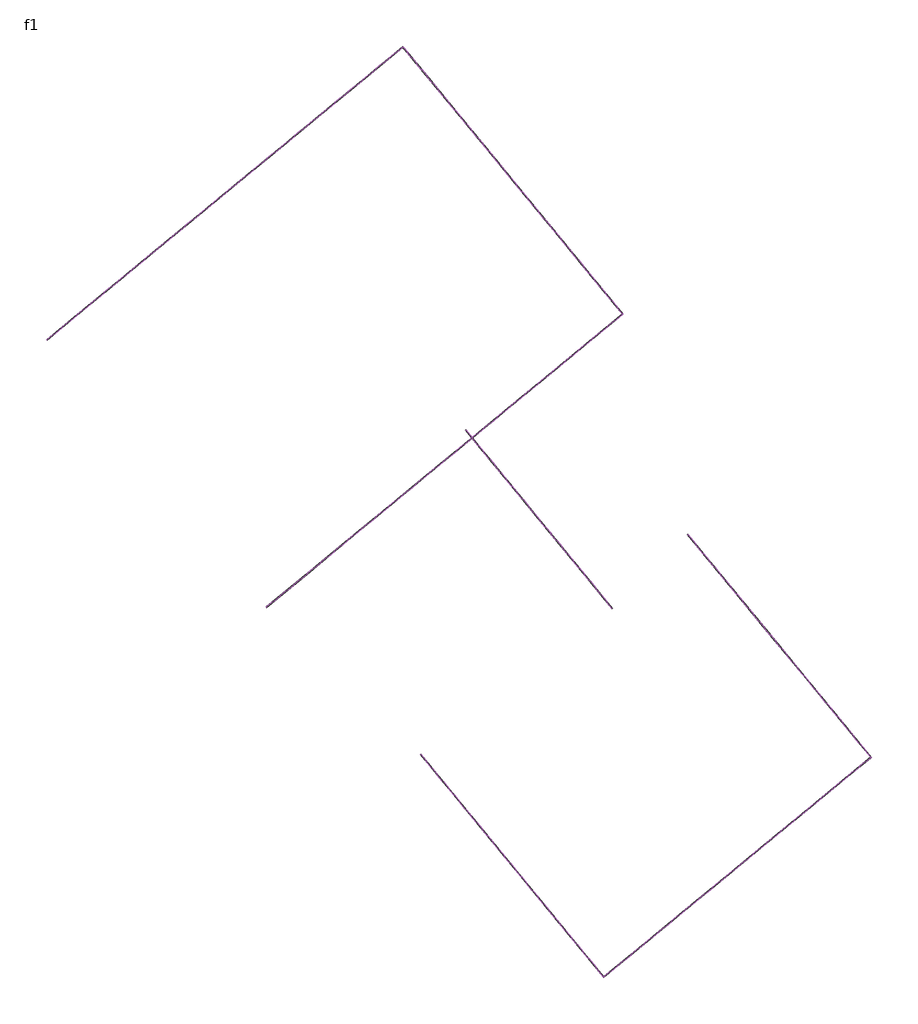
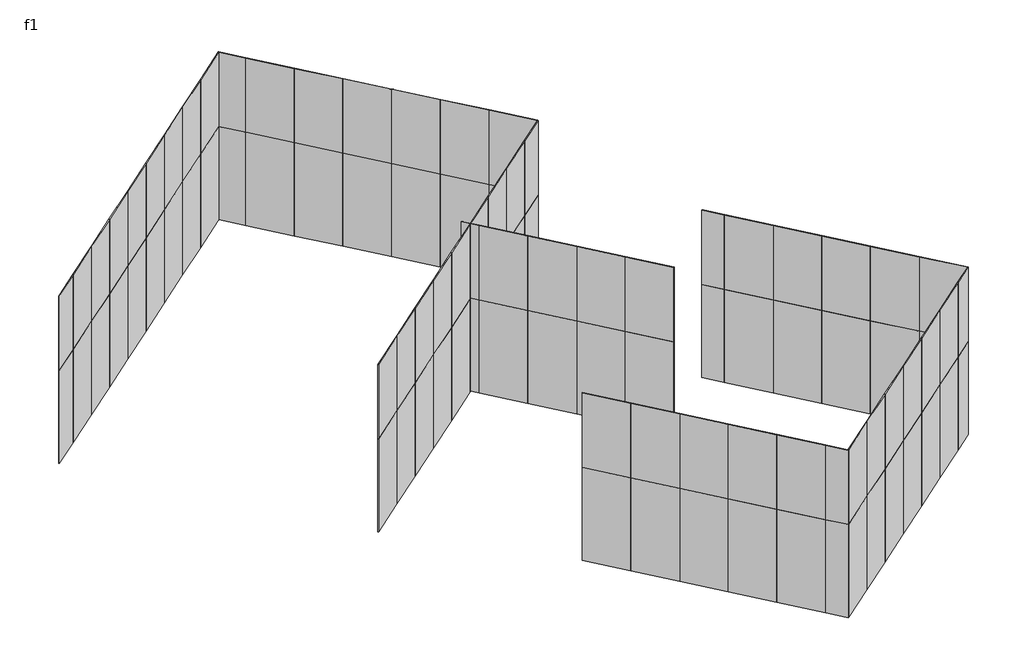
# One storey: 98 plates.
"""IFC4 building model written with IfcOpenShell, lengths in millimetres."""

import ifcopenshell
import ifcopenshell.guid

model = None  # the IFC model being written
_history = None  # IfcOwnerHistory: only IFC2X3 demands one
_inside = {}  # id of a spatial element -> (the spatial element, [elements in it])
_under = {}  # id of a project, library or spatial element -> (it, [spatial elements below it])
_declared = {}  # id of a project -> (the project, [libraries it declares])
_typed = {}  # id of a type object -> (the type object, [elements of that type])
_made_of = {}  # id of a material, layer set ... -> (it, [elements and type objects made of it])


def new_model(schema):
    """Start an empty IFC model of exactly this schema.

    Asked for "IFC4X3", IfcOpenShell would pick the latest addendum, in which some entities
    have other attributes; the version numbers below select the first issue.
    IFC2X3 requires an IfcOwnerHistory on every rooted entity: one is made here for all.
    """
    global model, _history
    if schema == "IFC4X3":
        model = ifcopenshell.file(schema_version=(4, 3, 0, 0))
    else:
        model = ifcopenshell.file(schema=schema)
    _inside.clear()
    _under.clear()
    _declared.clear()
    _typed.clear()
    _made_of.clear()
    _history = None
    if model.schema == "IFC2X3":
        org = make("IfcOrganization", Name="unknown")
        user = make(
            "IfcPersonAndOrganization",
            ThePerson=make("IfcPerson", FamilyName="unknown"),
            TheOrganization=org,
        )
        app = make(
            "IfcApplication",
            ApplicationDeveloper=org,
            Version="unknown",
            ApplicationFullName="unknown",
            ApplicationIdentifier="unknown",
        )
        _history = make(
            "IfcOwnerHistory",
            OwningUser=user,
            OwningApplication=app,
            ChangeAction="ADDED",
            CreationDate=0,
        )
    return model


def make(cls, **values):
    """One entity of the class cls with the attributes given. An attribute that is None is left unset."""
    return model.create_entity(
        cls, **{name: value for name, value in values.items() if value is not None}
    )


def rooted(cls, **values):
    """An entity with a GlobalId (a new one), such as an element, a storey or a relation."""
    return make(cls, GlobalId=ifcopenshell.guid.new(), OwnerHistory=_history, **values)


def si_unit(unit_type, name, prefix=None):
    """IfcSIUnit, for example si_unit("LENGTHUNIT", "METRE", prefix="MILLI")."""
    return make("IfcSIUnit", UnitType=unit_type, Prefix=prefix, Name=name)


def assignment(units):
    """IfcUnitAssignment: the units of a project."""
    return None if units is None else make("IfcUnitAssignment", Units=units)


def point(xyz):
    """IfcCartesianPoint."""
    return None if xyz is None else make("IfcCartesianPoint", Coordinates=xyz)


def direction(xyz):
    """IfcDirection."""
    return None if xyz is None else make("IfcDirection", DirectionRatios=xyz)


def frame(location, z_axis=None, x_axis=None):
    """IfcAxis2Placement3D, a coordinate frame: its origin and axes. An axis left out is left unset."""
    return make(
        "IfcAxis2Placement3D",
        Location=point(location),
        Axis=direction(z_axis),
        RefDirection=direction(x_axis),
    )


def origin():
    """The frame at (0, 0, 0) with its axes left unset."""
    return frame((0.0, 0.0, 0.0))


def origin_with_axes():
    """The frame at (0, 0, 0) with the z axis (0, 0, 1) and the x axis (1, 0, 0) written out."""
    return frame((0.0, 0.0, 0.0), z_axis=(0.0, 0.0, 1.0), x_axis=(1.0, 0.0, 0.0))


def place(relative_to, where):
    """IfcLocalPlacement: puts the frame where relative to a parent placement (None: the world)."""
    return make(
        "IfcLocalPlacement", PlacementRelTo=relative_to, RelativePlacement=where
    )


def context(
    kind, dimensions, precision=None, world=None, true_north=None, identifier=None
):
    """IfcGeometricRepresentationContext, for example the 3D "Model" context."""
    return make(
        "IfcGeometricRepresentationContext",
        ContextIdentifier=identifier,
        ContextType=kind,
        CoordinateSpaceDimension=dimensions,
        Precision=precision,
        WorldCoordinateSystem=world,
        TrueNorth=true_north,
    )


def project(units=None, contexts=None):
    """IfcProject with its units and contexts."""
    return rooted(
        "IfcProject",
        Name="project",
        RepresentationContexts=contexts,
        UnitsInContext=assignment(units),
    )


def spatial(cls, under=None, at=None, **own):
    """A site, building, storey or space (cls), placed at a placement, below another one or the project."""
    s = rooted(cls, ObjectPlacement=at, **own)
    if under is not None:
        _under.setdefault(under.id(), (under, []))[1].append(s)
    return s


def polyline(points):
    """IfcPolyline through the points."""
    return make("IfcPolyline", Points=[point(p) for p in points])


def outline(outer, holes=None, kind="AREA"):
    """IfcArbitraryClosedProfileDef: a profile drawn as a closed curve; with holes, ...WithVoids."""
    if holes is None:
        return make("IfcArbitraryClosedProfileDef", ProfileType=kind, OuterCurve=outer)
    return make(
        "IfcArbitraryProfileDefWithVoids",
        ProfileType=kind,
        OuterCurve=outer,
        InnerCurves=holes,
    )


def extrude(swept, where, along, depth):
    """IfcExtrudedAreaSolid: the profile swept, set in the frame where, extruded along a direction by depth."""
    return make(
        "IfcExtrudedAreaSolid",
        SweptArea=swept,
        Position=where,
        ExtrudedDirection=direction(along),
        Depth=depth,
    )


def shape(context_of_items, identifier, shape_type, items):
    """IfcShapeRepresentation: the items that make up one representation, for example the "Body"."""
    return make(
        "IfcShapeRepresentation",
        ContextOfItems=context_of_items,
        RepresentationIdentifier=identifier,
        RepresentationType=shape_type,
        Items=items,
    )


def source(mapping_origin, context_of_items, identifier, shape_type, items):
    """IfcRepresentationMap: a shape defined once, which mapped items show again and again."""
    return make(
        "IfcRepresentationMap",
        MappingOrigin=mapping_origin,
        MappedRepresentation=shape(context_of_items, identifier, shape_type, items),
    )


def transform(
    local_origin,
    x_axis=None,
    y_axis=None,
    z_axis=None,
    scale=None,
    scale2=None,
    scale3=None,
    uniform=True,
):
    """IfcCartesianTransformationOperator3D, or its non-uniform kind. x_axis, y_axis, z_axis: its Axis1, 2, 3."""
    if uniform:
        return make(
            "IfcCartesianTransformationOperator3D",
            Axis1=direction(x_axis),
            Axis2=direction(y_axis),
            LocalOrigin=point(local_origin),
            Scale=scale,
            Axis3=direction(z_axis),
        )
    return make(
        "IfcCartesianTransformationOperator3DnonUniform",
        Axis1=direction(x_axis),
        Axis2=direction(y_axis),
        LocalOrigin=point(local_origin),
        Scale=scale,
        Axis3=direction(z_axis),
        Scale2=scale2,
        Scale3=scale3,
    )


def mapped(mapping_source, mapping_target):
    """IfcMappedItem: shows the shape of a source again, moved by a transform."""
    return make(
        "IfcMappedItem", MappingSource=mapping_source, MappingTarget=mapping_target
    )


def made_of(thing, what):
    """Note that an element or type object is made of a material, layer set ...; save() writes the relation."""
    if what is not None:
        _made_of.setdefault(what.id(), (what, []))[1].append(thing)
    return thing


def element(
    cls,
    number,
    at=None,
    inside=None,
    cuts=None,
    type_object=None,
    material=None,
    context=None,
    identifier="Body",
    shape_type=None,
    held_by="IfcProductDefinitionShape",
    body=None,
    shapes=None,
    **own,
):
    """One element of the class cls, such as IfcWall. Its Tag is "e" and its number.

    at: its placement. inside: the storey or other place that contains it. cuts: it is an
    opening in that element (IfcRelVoidsElement). A single representation is given by context,
    identifier, shape_type and body (its items); several are given by shapes. held_by: the class
    of the entity that holds the representations. save() writes the other relations.
    """
    e = rooted(cls, Tag="e%d" % number, ObjectPlacement=at, **own)
    if body is not None:
        shapes = [shape(context, identifier, shape_type, body)]
    if shapes is not None:
        e.Representation = make(held_by, Representations=shapes)
    if inside is not None:
        _inside.setdefault(inside.id(), (inside, []))[1].append(e)
    if cuts is not None:
        rooted(
            "IfcRelVoidsElement", RelatingBuildingElement=cuts, RelatedOpeningElement=e
        )
    if type_object is not None:
        _typed.setdefault(type_object.id(), (type_object, []))[1].append(e)
    return made_of(e, material)


def aggregate(whole, parts):
    """IfcRelAggregates: a whole, such as a stair, and the parts it consists of."""
    return rooted("IfcRelAggregates", RelatingObject=whole, RelatedObjects=parts)


def save(model, path):
    """Write the relations noted so far, then the file.

    IfcRelAggregates (storeys below a building ...), IfcRelContainedInSpatialStructure (elements
    in a storey), IfcRelDefinesByType, IfcRelAssociatesMaterial and IfcRelDeclares: one each for
    every whole, place, type object, material and project.
    """
    for whole, parts in _under.values():
        aggregate(whole, parts)
    for where, things in _inside.values():
        rooted(
            "IfcRelContainedInSpatialStructure",
            RelatedElements=things,
            RelatingStructure=where,
        )
    for kind, things in _typed.values():
        rooted("IfcRelDefinesByType", RelatedObjects=things, RelatingType=kind)
    for what, things in _made_of.values():
        rooted("IfcRelAssociatesMaterial", RelatedObjects=things, RelatingMaterial=what)
    for by, libraries in _declared.values():
        rooted("IfcRelDeclares", RelatingContext=by, RelatedDefinitions=libraries)
    model.write(path)


def plate_0c29ff76(model_context):
    return source(origin(), model_context, "Body", "SweptSolid", [
        extrude(outline(polyline([(915.0, -12.5), (-915.0, -12.5), (-915.0, 12.5), (915.0, 12.5), (915.0, -12.5)])), origin_with_axes(), (0.0, 0.0, 1.0), 4000.0),
    ])


def plate_1e3715b7(model_context):
    return source(origin(), model_context, "Body", "SweptSolid", [
        extrude(outline(polyline([(510.0, -12.5), (-510.0, -12.5), (-510.0, 12.5), (510.0, 12.5), (510.0, -12.5)])), origin_with_axes(), (0.0, 0.0, 1.0), 4000.0),
    ])


def plate_751a20d5(model_context):
    return source(origin(), model_context, "Body", "SweptSolid", [
        extrude(outline(polyline([(915.0, -12.5), (-915.0, -12.5), (-915.0, 12.5), (915.0, 12.5), (915.0, -12.5)])), origin_with_axes(), (0.0, 0.0, 1.0), 3200.0),
    ])


def plate_eba9dd67(model_context):
    return source(origin(), model_context, "Body", "SweptSolid", [
        extrude(outline(polyline([(510.0, -12.5), (-510.0, -12.5), (-510.0, 12.5), (510.0, 12.5), (510.0, -12.5)])), origin_with_axes(), (0.0, 0.0, 1.0), 3200.0),
    ])


def plate_e4d7b700(model_context):
    return source(origin(), model_context, "Body", "SweptSolid", [
        extrude(outline(polyline([(680.0, -12.5), (-680.0, -12.5), (-680.0, 12.5), (680.0, 12.5), (680.0, -12.5)])), origin_with_axes(), (0.0, 0.0, 1.0), 4000.0),
    ])


def plate_81ff145c(model_context):
    return source(origin(), model_context, "Body", "SweptSolid", [
        extrude(outline(polyline([(680.0, -12.5), (-680.0, -12.5), (-680.0, 12.5), (680.0, 12.5), (680.0, -12.5)])), origin_with_axes(), (0.0, 0.0, 1.0), 3200.0),
    ])


def plate_147ead81(model_context):
    return source(origin(), model_context, "Body", "SweptSolid", [
        extrude(outline(polyline([(340.0, -12.5), (-340.0, -12.5), (-340.0, 12.5), (340.0, 12.5), (340.0, -12.5)])), origin_with_axes(), (0.0, 0.0, 1.0), 4000.0),
    ])


def plate_e10281fb(model_context):
    return source(origin(), model_context, "Body", "SweptSolid", [
        extrude(outline(polyline([(340.0, -12.5), (-340.0, -12.5), (-340.0, 12.5), (340.0, 12.5), (340.0, -12.5)])), origin_with_axes(), (0.0, 0.0, 1.0), 3200.0),
    ])


def plate_7a48b0fb(model_context):
    return source(origin(), model_context, "Body", "SweptSolid", [
        extrude(outline(polyline([(425.0, -12.5), (-425.0, -12.5), (-425.0, 12.5), (425.0, 12.5), (425.0, -12.5)])), origin_with_axes(), (0.0, 0.0, 1.0), 4000.0),
    ])


def plate_d5b4aa06(model_context):
    return source(origin(), model_context, "Body", "SweptSolid", [
        extrude(outline(polyline([(425.0, -12.5), (-425.0, -12.5), (-425.0, 12.5), (425.0, 12.5), (425.0, -12.5)])), origin_with_axes(), (0.0, 0.0, 1.0), 3200.0),
    ])


model = new_model("IFC4")

# Units and contexts
model_context = context("Model", 3, world=origin())
ifc_project = project(units=[si_unit("LENGTHUNIT", "METRE", prefix="MILLI")], contexts=[model_context])

# Site, building, storey
site = spatial("IfcSite", under=ifc_project)
building = spatial("IfcBuilding", under=site)
storey = spatial("IfcBuildingStorey", under=building, Name="f1", Elevation=3100.0)

# Plates
placement = place(None, origin())
plate_shape = plate_0c29ff76(model_context)
element("IfcPlate", 1, ObjectType="系统嵌板 : 玻璃", at=placement, inside=storey, context=model_context, shape_type="MappedRepresentation", body=[
    mapped(plate_shape, transform((-285.1263111, 24847.3639249, 3100.0), x_axis=(-0.6354332562848273, 0.7721557982734191, 0.0), y_axis=(-0.7721557982734191, -0.6354332562848273, 0.0), z_axis=(0.0, 0.0, 1.0))),
])
element("IfcPlate", 2, ObjectType="系统嵌板 : 玻璃", at=placement, inside=storey, context=model_context, shape_type="MappedRepresentation", body=[
    mapped(plate_shape, transform((-1447.9691701, 26260.4090358, 3100.0), x_axis=(-0.6354332562848273, 0.7721557982734191, 0.0), y_axis=(-0.7721557982734191, -0.6354332562848273, 0.0), z_axis=(0.0, 0.0, 1.0))),
])
element("IfcPlate", 3, ObjectType="系统嵌板 : 玻璃", at=placement, inside=storey, context=model_context, shape_type="MappedRepresentation", body=[
    mapped(plate_shape, transform((-2610.8120291, 27673.4541466, 3100.0), x_axis=(-0.6354332562848273, 0.7721557982734191, 0.0), y_axis=(-0.7721557982734191, -0.6354332562848273, 0.0), z_axis=(0.0, 0.0, 1.0))),
])
element("IfcPlate", 4, ObjectType="系统嵌板 : 玻璃", at=placement, inside=storey, context=model_context, shape_type="MappedRepresentation", body=[
    mapped(plate_shape, transform((-3773.6548881, 29086.4992575, 3100.0), x_axis=(-0.6354332562848273, 0.7721557982734191, 0.0), y_axis=(-0.7721557982734191, -0.6354332562848273, 0.0), z_axis=(0.0, 0.0, 1.0))),
])
element("IfcPlate", 5, ObjectType="系统嵌板 : 玻璃", at=placement, inside=storey, context=model_context, shape_type="MappedRepresentation", body=[
    mapped(plate_shape, transform((-4936.4977471, 30499.5443683, 3100.0), x_axis=(-0.6354332562848273, 0.7721557982734191, 0.0), y_axis=(-0.7721557982734191, -0.6354332562848273, 0.0), z_axis=(0.0, 0.0, 1.0))),
])
element("IfcPlate", 6, ObjectType="系统嵌板 : 玻璃", at=placement, inside=storey, context=model_context, shape_type="MappedRepresentation", body=[
    mapped(plate_shape, transform((-6099.3406061, 31912.5894791, 3100.0), x_axis=(-0.6354332562848273, 0.7721557982734191, 0.0), y_axis=(-0.7721557982734191, -0.6354332562848273, 0.0), z_axis=(0.0, 0.0, 1.0))),
])
element("IfcPlate", 7, ObjectType="系统嵌板 : 玻璃", at=placement, inside=storey, context=model_context, shape_type="MappedRepresentation", body=[
    mapped(plate_shape, transform((-8035.4265124, 32825.2895193, 3100.0), x_axis=(-0.7721557982734191, -0.6354332562848274, 0.0), y_axis=(0.6354332562848274, -0.7721557982734191, 0.0), z_axis=(0.0, 0.0, 1.0))),
])
element("IfcPlate", 8, ObjectType="系统嵌板 : 玻璃", at=placement, inside=storey, context=model_context, shape_type="MappedRepresentation", body=[
    mapped(plate_shape, transform((-9448.4716233, 31662.4466603, 3100.0), x_axis=(-0.7721557982734191, -0.6354332562848274, 0.0), y_axis=(0.6354332562848274, -0.7721557982734191, 0.0), z_axis=(0.0, 0.0, 1.0))),
])
element("IfcPlate", 9, ObjectType="系统嵌板 : 玻璃", at=placement, inside=storey, context=model_context, shape_type="MappedRepresentation", body=[
    mapped(plate_shape, transform((-10861.5167341, 30499.6038013, 3100.0), x_axis=(-0.7721557982734191, -0.6354332562848274, 0.0), y_axis=(0.6354332562848274, -0.7721557982734191, 0.0), z_axis=(0.0, 0.0, 1.0))),
])
element("IfcPlate", 10, ObjectType="系统嵌板 : 玻璃", at=placement, inside=storey, context=model_context, shape_type="MappedRepresentation", body=[
    mapped(plate_shape, transform((-12274.561845, 29336.7609423, 3100.0), x_axis=(-0.7721557982734191, -0.6354332562848274, 0.0), y_axis=(0.6354332562848274, -0.7721557982734191, 0.0), z_axis=(0.0, 0.0, 1.0))),
])
element("IfcPlate", 11, ObjectType="系统嵌板 : 玻璃", at=placement, inside=storey, context=model_context, shape_type="MappedRepresentation", body=[
    mapped(plate_shape, transform((-13687.6069558, 28173.9180833, 3100.0), x_axis=(-0.7721557982734191, -0.6354332562848274, 0.0), y_axis=(0.6354332562848274, -0.7721557982734191, 0.0), z_axis=(0.0, 0.0, 1.0))),
])
element("IfcPlate", 12, ObjectType="系统嵌板 : 玻璃", at=placement, inside=storey, context=model_context, shape_type="MappedRepresentation", body=[
    mapped(plate_shape, transform((-15100.6520666, 27011.0752243, 3100.0), x_axis=(-0.7721557982734191, -0.6354332562848274, 0.0), y_axis=(0.6354332562848274, -0.7721557982734191, 0.0), z_axis=(0.0, 0.0, 1.0))),
])
element("IfcPlate", 13, ObjectType="系统嵌板 : 玻璃", at=placement, inside=storey, context=model_context, shape_type="MappedRepresentation", body=[
    mapped(plate_shape, transform((-16513.6971775, 25848.2323653, 3100.0), x_axis=(-0.7721557982734191, -0.6354332562848274, 0.0), y_axis=(0.6354332562848274, -0.7721557982734191, 0.0), z_axis=(0.0, 0.0, 1.0))),
])
element("IfcPlate", 14, ObjectType="系统嵌板 : 玻璃", at=placement, inside=storey, context=model_context, shape_type="MappedRepresentation", body=[
    mapped(plate_shape, transform((-17926.7422883, 24685.3895063, 3100.0), x_axis=(-0.7721557982734191, -0.6354332562848274, 0.0), y_axis=(0.6354332562848274, -0.7721557982734191, 0.0), z_axis=(0.0, 0.0, 1.0))),
])
element("IfcPlate", 15, ObjectType="系统嵌板 : 玻璃", at=placement, inside=storey, context=model_context, shape_type="MappedRepresentation", body=[
    mapped(plate_shape, transform((-11351.6750986, 14555.3306985, 3100.0), x_axis=(0.772155798273419, 0.6354332562848274, 0.0), y_axis=(-0.6354332562848274, 0.772155798273419, 0.0), z_axis=(0.0, 0.0, 1.0))),
])
element("IfcPlate", 16, ObjectType="系统嵌板 : 玻璃", at=placement, inside=storey, context=model_context, shape_type="MappedRepresentation", body=[
    mapped(plate_shape, transform((-9938.6299877, 15718.1735575, 3100.0), x_axis=(0.772155798273419, 0.6354332562848274, 0.0), y_axis=(-0.6354332562848274, 0.772155798273419, 0.0), z_axis=(0.0, 0.0, 1.0))),
])
element("IfcPlate", 17, ObjectType="系统嵌板 : 玻璃", at=placement, inside=storey, context=model_context, shape_type="MappedRepresentation", body=[
    mapped(plate_shape, transform((-8525.5848769, 16881.0164165, 3100.0), x_axis=(0.772155798273419, 0.6354332562848274, 0.0), y_axis=(-0.6354332562848274, 0.772155798273419, 0.0), z_axis=(0.0, 0.0, 1.0))),
])
element("IfcPlate", 18, ObjectType="系统嵌板 : 玻璃", at=placement, inside=storey, context=model_context, shape_type="MappedRepresentation", body=[
    mapped(plate_shape, transform((-7112.539766, 18043.8592755, 3100.0), x_axis=(0.772155798273419, 0.6354332562848274, 0.0), y_axis=(-0.6354332562848274, 0.772155798273419, 0.0), z_axis=(0.0, 0.0, 1.0))),
])
element("IfcPlate", 19, ObjectType="系统嵌板 : 玻璃", at=placement, inside=storey, context=model_context, shape_type="MappedRepresentation", body=[
    mapped(plate_shape, transform((-5699.4946552, 19206.7021345, 3100.0), x_axis=(0.772155798273419, 0.6354332562848274, 0.0), y_axis=(-0.6354332562848274, 0.772155798273419, 0.0), z_axis=(0.0, 0.0, 1.0))),
])
element("IfcPlate", 20, ObjectType="系统嵌板 : 玻璃", at=placement, inside=storey, context=model_context, shape_type="MappedRepresentation", body=[
    mapped(plate_shape, transform((-4286.4495444, 20369.5449935, 3100.0), x_axis=(0.772155798273419, 0.6354332562848274, 0.0), y_axis=(-0.6354332562848274, 0.772155798273419, 0.0), z_axis=(0.0, 0.0, 1.0))),
])
element("IfcPlate", 21, ObjectType="系统嵌板 : 玻璃", at=placement, inside=storey, context=model_context, shape_type="MappedRepresentation", body=[
    mapped(plate_shape, transform((-2873.4044335, 21532.3878525, 3100.0), x_axis=(0.772155798273419, 0.6354332562848274, 0.0), y_axis=(-0.6354332562848274, 0.772155798273419, 0.0), z_axis=(0.0, 0.0, 1.0))),
])
element("IfcPlate", 22, ObjectType="系统嵌板 : 玻璃", at=placement, inside=storey, context=model_context, shape_type="MappedRepresentation", body=[
    mapped(plate_shape, transform((-1460.3593227, 22695.2307115, 3100.0), x_axis=(0.772155798273419, 0.6354332562848274, 0.0), y_axis=(-0.6354332562848274, 0.772155798273419, 0.0), z_axis=(0.0, 0.0, 1.0))),
])
element("IfcPlate", 23, ObjectType="系统嵌板 : 玻璃", at=placement, inside=storey, context=model_context, shape_type="MappedRepresentation", body=[
    mapped(plate_shape, transform((-640.1697835, 14643.621577, 3100.0), x_axis=(-0.6354332562848286, 0.7721557982734181, 0.0), y_axis=(-0.7721557982734181, -0.6354332562848286, 0.0), z_axis=(0.0, 0.0, 1.0))),
])
element("IfcPlate", 24, ObjectType="系统嵌板 : 玻璃", at=placement, inside=storey, context=model_context, shape_type="MappedRepresentation", body=[
    mapped(plate_shape, transform((-1803.0126425, 16056.6666878, 3100.0), x_axis=(-0.6354332562848286, 0.7721557982734181, 0.0), y_axis=(-0.7721557982734181, -0.6354332562848286, 0.0), z_axis=(0.0, 0.0, 1.0))),
])
element("IfcPlate", 25, ObjectType="系统嵌板 : 玻璃", at=placement, inside=storey, context=model_context, shape_type="MappedRepresentation", body=[
    mapped(plate_shape, transform((-2965.8555015, 17469.7117987, 3100.0), x_axis=(-0.6354332562848286, 0.7721557982734181, 0.0), y_axis=(-0.7721557982734181, -0.6354332562848286, 0.0), z_axis=(0.0, 0.0, 1.0))),
])
element("IfcPlate", 26, ObjectType="系统嵌板 : 玻璃", at=placement, inside=storey, context=model_context, shape_type="MappedRepresentation", body=[
    mapped(plate_shape, transform((-4128.6983605, 18882.7569095, 3100.0), x_axis=(-0.6354332562848286, 0.7721557982734181, 0.0), y_axis=(-0.7721557982734181, -0.6354332562848286, 0.0), z_axis=(0.0, 0.0, 1.0))),
])
element("IfcPlate", 27, ObjectType="系统嵌板 : 玻璃", at=placement, inside=storey, context=model_context, shape_type="MappedRepresentation", body=[
    mapped(plate_shape, transform((8328.6158526, 9478.9823292, 3100.0), x_axis=(-0.6354332562848274, 0.772155798273419, 0.0), y_axis=(-0.772155798273419, -0.6354332562848274, 0.0), z_axis=(0.0, 0.0, 1.0))),
])
element("IfcPlate", 28, ObjectType="系统嵌板 : 玻璃", at=placement, inside=storey, context=model_context, shape_type="MappedRepresentation", body=[
    mapped(plate_shape, transform((7165.7729936, 10892.02744, 3100.0), x_axis=(-0.6354332562848274, 0.772155798273419, 0.0), y_axis=(-0.772155798273419, -0.6354332562848274, 0.0), z_axis=(0.0, 0.0, 1.0))),
])
element("IfcPlate", 29, ObjectType="系统嵌板 : 玻璃", at=placement, inside=storey, context=model_context, shape_type="MappedRepresentation", body=[
    mapped(plate_shape, transform((6002.9301346, 12305.0725508, 3100.0), x_axis=(-0.6354332562848274, 0.772155798273419, 0.0), y_axis=(-0.772155798273419, -0.6354332562848274, 0.0), z_axis=(0.0, 0.0, 1.0))),
])
element("IfcPlate", 30, ObjectType="系统嵌板 : 玻璃", at=placement, inside=storey, context=model_context, shape_type="MappedRepresentation", body=[
    mapped(plate_shape, transform((4840.0872756, 13718.1176617, 3100.0), x_axis=(-0.6354332562848274, 0.772155798273419, 0.0), y_axis=(-0.772155798273419, -0.6354332562848274, 0.0), z_axis=(0.0, 0.0, 1.0))),
])
element("IfcPlate", 31, ObjectType="系统嵌板 : 玻璃", at=placement, inside=storey, context=model_context, shape_type="MappedRepresentation", body=[
    mapped(plate_shape, transform((3677.2444166, 15131.1627725, 3100.0), x_axis=(-0.6354332562848274, 0.772155798273419, 0.0), y_axis=(-0.772155798273419, -0.6354332562848274, 0.0), z_axis=(0.0, 0.0, 1.0))),
])
element("IfcPlate", 32, ObjectType="系统嵌板 : 玻璃", at=placement, inside=storey, context=model_context, shape_type="MappedRepresentation", body=[
    mapped(plate_shape, transform((350.6902583, 1728.6821278, 3100.0), x_axis=(0.7721557982734191, 0.6354332562848273, 0.0), y_axis=(-0.6354332562848273, 0.7721557982734191, 0.0), z_axis=(0.0, 0.0, 1.0))),
])
element("IfcPlate", 33, ObjectType="系统嵌板 : 玻璃", at=placement, inside=storey, context=model_context, shape_type="MappedRepresentation", body=[
    mapped(plate_shape, transform((1763.7353691, 2891.5249868, 3100.0), x_axis=(0.7721557982734191, 0.6354332562848273, 0.0), y_axis=(-0.6354332562848273, 0.7721557982734191, 0.0), z_axis=(0.0, 0.0, 1.0))),
])
element("IfcPlate", 34, ObjectType="系统嵌板 : 玻璃", at=placement, inside=storey, context=model_context, shape_type="MappedRepresentation", body=[
    mapped(plate_shape, transform((3176.78048, 4054.3678458, 3100.0), x_axis=(0.7721557982734191, 0.6354332562848273, 0.0), y_axis=(-0.6354332562848273, 0.7721557982734191, 0.0), z_axis=(0.0, 0.0, 1.0))),
])
element("IfcPlate", 35, ObjectType="系统嵌板 : 玻璃", at=placement, inside=storey, context=model_context, shape_type="MappedRepresentation", body=[
    mapped(plate_shape, transform((4589.8255908, 5217.2107048, 3100.0), x_axis=(0.7721557982734191, 0.6354332562848273, 0.0), y_axis=(-0.6354332562848273, 0.7721557982734191, 0.0), z_axis=(0.0, 0.0, 1.0))),
])
element("IfcPlate", 36, ObjectType="系统嵌板 : 玻璃", at=placement, inside=storey, context=model_context, shape_type="MappedRepresentation", body=[
    mapped(plate_shape, transform((6002.8707016, 6380.0535638, 3100.0), x_axis=(0.7721557982734191, 0.6354332562848273, 0.0), y_axis=(-0.6354332562848273, 0.7721557982734191, 0.0), z_axis=(0.0, 0.0, 1.0))),
])
element("IfcPlate", 37, ObjectType="系统嵌板 : 玻璃", at=placement, inside=storey, context=model_context, shape_type="MappedRepresentation", body=[
    mapped(plate_shape, transform((7415.9158125, 7542.8964228, 3100.0), x_axis=(0.7721557982734191, 0.6354332562848273, 0.0), y_axis=(-0.6354332562848273, 0.7721557982734191, 0.0), z_axis=(0.0, 0.0, 1.0))),
])
element("IfcPlate", 38, ObjectType="系统嵌板 : 玻璃", at=placement, inside=storey, context=model_context, shape_type="MappedRepresentation", body=[
    mapped(plate_shape, transform((-6128.7434305, 8162.2961256, 3100.0), x_axis=(0.6354332562848274, -0.7721557982734191, 0.0), y_axis=(0.7721557982734191, 0.6354332562848274, 0.0), z_axis=(0.0, 0.0, 1.0))),
])
element("IfcPlate", 39, ObjectType="系统嵌板 : 玻璃", at=placement, inside=storey, context=model_context, shape_type="MappedRepresentation", body=[
    mapped(plate_shape, transform((-4965.9005715, 6749.2510148, 3100.0), x_axis=(0.6354332562848274, -0.7721557982734191, 0.0), y_axis=(0.7721557982734191, 0.6354332562848274, 0.0), z_axis=(0.0, 0.0, 1.0))),
])
element("IfcPlate", 40, ObjectType="系统嵌板 : 玻璃", at=placement, inside=storey, context=model_context, shape_type="MappedRepresentation", body=[
    mapped(plate_shape, transform((-3803.0577125, 5336.2059039, 3100.0), x_axis=(0.6354332562848274, -0.7721557982734191, 0.0), y_axis=(0.7721557982734191, 0.6354332562848274, 0.0), z_axis=(0.0, 0.0, 1.0))),
])
element("IfcPlate", 41, ObjectType="系统嵌板 : 玻璃", at=placement, inside=storey, context=model_context, shape_type="MappedRepresentation", body=[
    mapped(plate_shape, transform((-2640.2148535, 3923.1607931, 3100.0), x_axis=(0.6354332562848274, -0.7721557982734191, 0.0), y_axis=(0.7721557982734191, 0.6354332562848274, 0.0), z_axis=(0.0, 0.0, 1.0))),
])
element("IfcPlate", 42, ObjectType="系统嵌板 : 玻璃", at=placement, inside=storey, context=model_context, shape_type="MappedRepresentation", body=[
    mapped(plate_shape, transform((-1477.3719945, 2510.1156823, 3100.0), x_axis=(0.6354332562848274, -0.7721557982734191, 0.0), y_axis=(0.7721557982734191, 0.6354332562848274, 0.0), z_axis=(0.0, 0.0, 1.0))),
])
plate_2_shape = plate_1e3715b7(model_context)
element("IfcPlate", 43, ObjectType="系统嵌板 : 玻璃", at=placement, inside=storey, context=model_context, shape_type="MappedRepresentation", body=[
    mapped(plate_2_shape, transform((-7004.8329963, 33012.9114917, 3100.0), x_axis=(-0.6354332562848273, 0.7721557982734191, 0.0), y_axis=(-0.7721557982734191, -0.6354332562848273, 0.0), z_axis=(0.0, 0.0, 1.0))),
])
element("IfcPlate", 44, ObjectType="系统嵌板 : 玻璃", at=placement, inside=storey, context=model_context, shape_type="MappedRepresentation", body=[
    mapped(plate_2_shape, transform((8516.237825, 8448.388813, 3100.0), x_axis=(0.7721557982734191, 0.6354332562848273, 0.0), y_axis=(-0.6354332562848273, 0.7721557982734191, 0.0), z_axis=(0.0, 0.0, 1.0))),
])
plate_3_shape = plate_751a20d5(model_context)
element("IfcPlate", 45, ObjectType="系统嵌板 : 玻璃", at=placement, inside=storey, context=model_context, shape_type="MappedRepresentation", body=[
    mapped(plate_3_shape, transform((-285.1263111, 24847.3639249, 7100.0), x_axis=(-0.6354332562848273, 0.7721557982734191, 0.0), y_axis=(-0.7721557982734191, -0.6354332562848273, 0.0), z_axis=(0.0, 0.0, 1.0))),
])
element("IfcPlate", 46, ObjectType="系统嵌板 : 玻璃", at=placement, inside=storey, context=model_context, shape_type="MappedRepresentation", body=[
    mapped(plate_3_shape, transform((-1447.9691701, 26260.4090358, 7100.0), x_axis=(-0.6354332562848273, 0.7721557982734191, 0.0), y_axis=(-0.7721557982734191, -0.6354332562848273, 0.0), z_axis=(0.0, 0.0, 1.0))),
])
element("IfcPlate", 47, ObjectType="系统嵌板 : 玻璃", at=placement, inside=storey, context=model_context, shape_type="MappedRepresentation", body=[
    mapped(plate_3_shape, transform((-2610.8120291, 27673.4541466, 7100.0), x_axis=(-0.6354332562848273, 0.7721557982734191, 0.0), y_axis=(-0.7721557982734191, -0.6354332562848273, 0.0), z_axis=(0.0, 0.0, 1.0))),
])
element("IfcPlate", 48, ObjectType="系统嵌板 : 玻璃", at=placement, inside=storey, context=model_context, shape_type="MappedRepresentation", body=[
    mapped(plate_3_shape, transform((-3773.6548881, 29086.4992575, 7100.0), x_axis=(-0.6354332562848273, 0.7721557982734191, 0.0), y_axis=(-0.7721557982734191, -0.6354332562848273, 0.0), z_axis=(0.0, 0.0, 1.0))),
])
element("IfcPlate", 49, ObjectType="系统嵌板 : 玻璃", at=placement, inside=storey, context=model_context, shape_type="MappedRepresentation", body=[
    mapped(plate_3_shape, transform((-4936.4977471, 30499.5443683, 7100.0), x_axis=(-0.6354332562848273, 0.7721557982734191, 0.0), y_axis=(-0.7721557982734191, -0.6354332562848273, 0.0), z_axis=(0.0, 0.0, 1.0))),
])
element("IfcPlate", 50, ObjectType="系统嵌板 : 玻璃", at=placement, inside=storey, context=model_context, shape_type="MappedRepresentation", body=[
    mapped(plate_3_shape, transform((-6099.3406061, 31912.5894791, 7100.0), x_axis=(-0.6354332562848273, 0.7721557982734191, 0.0), y_axis=(-0.7721557982734191, -0.6354332562848273, 0.0), z_axis=(0.0, 0.0, 1.0))),
])
element("IfcPlate", 51, ObjectType="系统嵌板 : 玻璃", at=placement, inside=storey, context=model_context, shape_type="MappedRepresentation", body=[
    mapped(plate_3_shape, transform((-8035.4265124, 32825.2895193, 7100.0), x_axis=(-0.7721557982734191, -0.6354332562848274, 0.0), y_axis=(0.6354332562848274, -0.7721557982734191, 0.0), z_axis=(0.0, 0.0, 1.0))),
])
element("IfcPlate", 52, ObjectType="系统嵌板 : 玻璃", at=placement, inside=storey, context=model_context, shape_type="MappedRepresentation", body=[
    mapped(plate_3_shape, transform((-9448.4716233, 31662.4466603, 7100.0), x_axis=(-0.7721557982734191, -0.6354332562848274, 0.0), y_axis=(0.6354332562848274, -0.7721557982734191, 0.0), z_axis=(0.0, 0.0, 1.0))),
])
element("IfcPlate", 53, ObjectType="系统嵌板 : 玻璃", at=placement, inside=storey, context=model_context, shape_type="MappedRepresentation", body=[
    mapped(plate_3_shape, transform((-10861.5167341, 30499.6038013, 7100.0), x_axis=(-0.7721557982734191, -0.6354332562848274, 0.0), y_axis=(0.6354332562848274, -0.7721557982734191, 0.0), z_axis=(0.0, 0.0, 1.0))),
])
element("IfcPlate", 54, ObjectType="系统嵌板 : 玻璃", at=placement, inside=storey, context=model_context, shape_type="MappedRepresentation", body=[
    mapped(plate_3_shape, transform((-12274.561845, 29336.7609423, 7100.0), x_axis=(-0.7721557982734191, -0.6354332562848274, 0.0), y_axis=(0.6354332562848274, -0.7721557982734191, 0.0), z_axis=(0.0, 0.0, 1.0))),
])
element("IfcPlate", 55, ObjectType="系统嵌板 : 玻璃", at=placement, inside=storey, context=model_context, shape_type="MappedRepresentation", body=[
    mapped(plate_3_shape, transform((-13687.6069558, 28173.9180833, 7100.0), x_axis=(-0.7721557982734191, -0.6354332562848274, 0.0), y_axis=(0.6354332562848274, -0.7721557982734191, 0.0), z_axis=(0.0, 0.0, 1.0))),
])
element("IfcPlate", 56, ObjectType="系统嵌板 : 玻璃", at=placement, inside=storey, context=model_context, shape_type="MappedRepresentation", body=[
    mapped(plate_3_shape, transform((-15100.6520666, 27011.0752243, 7100.0), x_axis=(-0.7721557982734191, -0.6354332562848274, 0.0), y_axis=(0.6354332562848274, -0.7721557982734191, 0.0), z_axis=(0.0, 0.0, 1.0))),
])
element("IfcPlate", 57, ObjectType="系统嵌板 : 玻璃", at=placement, inside=storey, context=model_context, shape_type="MappedRepresentation", body=[
    mapped(plate_3_shape, transform((-16513.6971775, 25848.2323653, 7100.0), x_axis=(-0.7721557982734191, -0.6354332562848274, 0.0), y_axis=(0.6354332562848274, -0.7721557982734191, 0.0), z_axis=(0.0, 0.0, 1.0))),
])
element("IfcPlate", 58, ObjectType="系统嵌板 : 玻璃", at=placement, inside=storey, context=model_context, shape_type="MappedRepresentation", body=[
    mapped(plate_3_shape, transform((-17926.7422883, 24685.3895063, 7100.0), x_axis=(-0.7721557982734191, -0.6354332562848274, 0.0), y_axis=(0.6354332562848274, -0.7721557982734191, 0.0), z_axis=(0.0, 0.0, 1.0))),
])
element("IfcPlate", 59, ObjectType="系统嵌板 : 玻璃", at=placement, inside=storey, context=model_context, shape_type="MappedRepresentation", body=[
    mapped(plate_3_shape, transform((-11351.6750986, 14555.3306985, 7100.0), x_axis=(0.772155798273419, 0.6354332562848274, 0.0), y_axis=(-0.6354332562848274, 0.772155798273419, 0.0), z_axis=(0.0, 0.0, 1.0))),
])
element("IfcPlate", 60, ObjectType="系统嵌板 : 玻璃", at=placement, inside=storey, context=model_context, shape_type="MappedRepresentation", body=[
    mapped(plate_3_shape, transform((-9938.6299877, 15718.1735575, 7100.0), x_axis=(0.772155798273419, 0.6354332562848274, 0.0), y_axis=(-0.6354332562848274, 0.772155798273419, 0.0), z_axis=(0.0, 0.0, 1.0))),
])
element("IfcPlate", 61, ObjectType="系统嵌板 : 玻璃", at=placement, inside=storey, context=model_context, shape_type="MappedRepresentation", body=[
    mapped(plate_3_shape, transform((-8525.5848769, 16881.0164165, 7100.0), x_axis=(0.772155798273419, 0.6354332562848274, 0.0), y_axis=(-0.6354332562848274, 0.772155798273419, 0.0), z_axis=(0.0, 0.0, 1.0))),
])
element("IfcPlate", 62, ObjectType="系统嵌板 : 玻璃", at=placement, inside=storey, context=model_context, shape_type="MappedRepresentation", body=[
    mapped(plate_3_shape, transform((-7112.539766, 18043.8592755, 7100.0), x_axis=(0.772155798273419, 0.6354332562848274, 0.0), y_axis=(-0.6354332562848274, 0.772155798273419, 0.0), z_axis=(0.0, 0.0, 1.0))),
])
element("IfcPlate", 63, ObjectType="系统嵌板 : 玻璃", at=placement, inside=storey, context=model_context, shape_type="MappedRepresentation", body=[
    mapped(plate_3_shape, transform((-5699.4946552, 19206.7021345, 7100.0), x_axis=(0.772155798273419, 0.6354332562848274, 0.0), y_axis=(-0.6354332562848274, 0.772155798273419, 0.0), z_axis=(0.0, 0.0, 1.0))),
])
element("IfcPlate", 64, ObjectType="系统嵌板 : 玻璃", at=placement, inside=storey, context=model_context, shape_type="MappedRepresentation", body=[
    mapped(plate_3_shape, transform((-4286.4495444, 20369.5449935, 7100.0), x_axis=(0.772155798273419, 0.6354332562848274, 0.0), y_axis=(-0.6354332562848274, 0.772155798273419, 0.0), z_axis=(0.0, 0.0, 1.0))),
])
element("IfcPlate", 65, ObjectType="系统嵌板 : 玻璃", at=placement, inside=storey, context=model_context, shape_type="MappedRepresentation", body=[
    mapped(plate_3_shape, transform((-2873.4044335, 21532.3878525, 7100.0), x_axis=(0.772155798273419, 0.6354332562848274, 0.0), y_axis=(-0.6354332562848274, 0.772155798273419, 0.0), z_axis=(0.0, 0.0, 1.0))),
])
element("IfcPlate", 66, ObjectType="系统嵌板 : 玻璃", at=placement, inside=storey, context=model_context, shape_type="MappedRepresentation", body=[
    mapped(plate_3_shape, transform((-1460.3593227, 22695.2307115, 7100.0), x_axis=(0.772155798273419, 0.6354332562848274, 0.0), y_axis=(-0.6354332562848274, 0.772155798273419, 0.0), z_axis=(0.0, 0.0, 1.0))),
])
element("IfcPlate", 67, ObjectType="系统嵌板 : 玻璃", at=placement, inside=storey, context=model_context, shape_type="MappedRepresentation", body=[
    mapped(plate_3_shape, transform((-640.1697835, 14643.621577, 7100.0), x_axis=(-0.6354332562848286, 0.7721557982734181, 0.0), y_axis=(-0.7721557982734181, -0.6354332562848286, 0.0), z_axis=(0.0, 0.0, 1.0))),
])
element("IfcPlate", 68, ObjectType="系统嵌板 : 玻璃", at=placement, inside=storey, context=model_context, shape_type="MappedRepresentation", body=[
    mapped(plate_3_shape, transform((-1803.0126425, 16056.6666878, 7100.0), x_axis=(-0.6354332562848286, 0.7721557982734181, 0.0), y_axis=(-0.7721557982734181, -0.6354332562848286, 0.0), z_axis=(0.0, 0.0, 1.0))),
])
element("IfcPlate", 69, ObjectType="系统嵌板 : 玻璃", at=placement, inside=storey, context=model_context, shape_type="MappedRepresentation", body=[
    mapped(plate_3_shape, transform((-2965.8555015, 17469.7117987, 7100.0), x_axis=(-0.6354332562848286, 0.7721557982734181, 0.0), y_axis=(-0.7721557982734181, -0.6354332562848286, 0.0), z_axis=(0.0, 0.0, 1.0))),
])
element("IfcPlate", 70, ObjectType="系统嵌板 : 玻璃", at=placement, inside=storey, context=model_context, shape_type="MappedRepresentation", body=[
    mapped(plate_3_shape, transform((-4128.6983605, 18882.7569095, 7100.0), x_axis=(-0.6354332562848286, 0.7721557982734181, 0.0), y_axis=(-0.7721557982734181, -0.6354332562848286, 0.0), z_axis=(0.0, 0.0, 1.0))),
])
element("IfcPlate", 71, ObjectType="系统嵌板 : 玻璃", at=placement, inside=storey, context=model_context, shape_type="MappedRepresentation", body=[
    mapped(plate_3_shape, transform((8328.6158526, 9478.9823292, 7100.0), x_axis=(-0.6354332562848274, 0.772155798273419, 0.0), y_axis=(-0.772155798273419, -0.6354332562848274, 0.0), z_axis=(0.0, 0.0, 1.0))),
])
element("IfcPlate", 72, ObjectType="系统嵌板 : 玻璃", at=placement, inside=storey, context=model_context, shape_type="MappedRepresentation", body=[
    mapped(plate_3_shape, transform((7165.7729936, 10892.02744, 7100.0), x_axis=(-0.6354332562848274, 0.772155798273419, 0.0), y_axis=(-0.772155798273419, -0.6354332562848274, 0.0), z_axis=(0.0, 0.0, 1.0))),
])
element("IfcPlate", 73, ObjectType="系统嵌板 : 玻璃", at=placement, inside=storey, context=model_context, shape_type="MappedRepresentation", body=[
    mapped(plate_3_shape, transform((6002.9301346, 12305.0725508, 7100.0), x_axis=(-0.6354332562848274, 0.772155798273419, 0.0), y_axis=(-0.772155798273419, -0.6354332562848274, 0.0), z_axis=(0.0, 0.0, 1.0))),
])
element("IfcPlate", 74, ObjectType="系统嵌板 : 玻璃", at=placement, inside=storey, context=model_context, shape_type="MappedRepresentation", body=[
    mapped(plate_3_shape, transform((4840.0872756, 13718.1176617, 7100.0), x_axis=(-0.6354332562848274, 0.772155798273419, 0.0), y_axis=(-0.772155798273419, -0.6354332562848274, 0.0), z_axis=(0.0, 0.0, 1.0))),
])
element("IfcPlate", 75, ObjectType="系统嵌板 : 玻璃", at=placement, inside=storey, context=model_context, shape_type="MappedRepresentation", body=[
    mapped(plate_3_shape, transform((3677.2444166, 15131.1627725, 7100.0), x_axis=(-0.6354332562848274, 0.772155798273419, 0.0), y_axis=(-0.772155798273419, -0.6354332562848274, 0.0), z_axis=(0.0, 0.0, 1.0))),
])
element("IfcPlate", 76, ObjectType="系统嵌板 : 玻璃", at=placement, inside=storey, context=model_context, shape_type="MappedRepresentation", body=[
    mapped(plate_3_shape, transform((350.6902583, 1728.6821278, 7100.0), x_axis=(0.7721557982734191, 0.6354332562848273, 0.0), y_axis=(-0.6354332562848273, 0.7721557982734191, 0.0), z_axis=(0.0, 0.0, 1.0))),
])
element("IfcPlate", 77, ObjectType="系统嵌板 : 玻璃", at=placement, inside=storey, context=model_context, shape_type="MappedRepresentation", body=[
    mapped(plate_3_shape, transform((1763.7353691, 2891.5249868, 7100.0), x_axis=(0.7721557982734191, 0.6354332562848273, 0.0), y_axis=(-0.6354332562848273, 0.7721557982734191, 0.0), z_axis=(0.0, 0.0, 1.0))),
])
element("IfcPlate", 78, ObjectType="系统嵌板 : 玻璃", at=placement, inside=storey, context=model_context, shape_type="MappedRepresentation", body=[
    mapped(plate_3_shape, transform((3176.78048, 4054.3678458, 7100.0), x_axis=(0.7721557982734191, 0.6354332562848273, 0.0), y_axis=(-0.6354332562848273, 0.7721557982734191, 0.0), z_axis=(0.0, 0.0, 1.0))),
])
element("IfcPlate", 79, ObjectType="系统嵌板 : 玻璃", at=placement, inside=storey, context=model_context, shape_type="MappedRepresentation", body=[
    mapped(plate_3_shape, transform((4589.8255908, 5217.2107048, 7100.0), x_axis=(0.7721557982734191, 0.6354332562848273, 0.0), y_axis=(-0.6354332562848273, 0.7721557982734191, 0.0), z_axis=(0.0, 0.0, 1.0))),
])
element("IfcPlate", 80, ObjectType="系统嵌板 : 玻璃", at=placement, inside=storey, context=model_context, shape_type="MappedRepresentation", body=[
    mapped(plate_3_shape, transform((6002.8707016, 6380.0535638, 7100.0), x_axis=(0.7721557982734191, 0.6354332562848273, 0.0), y_axis=(-0.6354332562848273, 0.7721557982734191, 0.0), z_axis=(0.0, 0.0, 1.0))),
])
element("IfcPlate", 81, ObjectType="系统嵌板 : 玻璃", at=placement, inside=storey, context=model_context, shape_type="MappedRepresentation", body=[
    mapped(plate_3_shape, transform((7415.9158125, 7542.8964228, 7100.0), x_axis=(0.7721557982734191, 0.6354332562848273, 0.0), y_axis=(-0.6354332562848273, 0.7721557982734191, 0.0), z_axis=(0.0, 0.0, 1.0))),
])
element("IfcPlate", 82, ObjectType="系统嵌板 : 玻璃", at=placement, inside=storey, context=model_context, shape_type="MappedRepresentation", body=[
    mapped(plate_3_shape, transform((-6128.7434305, 8162.2961256, 7100.0), x_axis=(0.6354332562848274, -0.7721557982734191, 0.0), y_axis=(0.7721557982734191, 0.6354332562848274, 0.0), z_axis=(0.0, 0.0, 1.0))),
])
element("IfcPlate", 83, ObjectType="系统嵌板 : 玻璃", at=placement, inside=storey, context=model_context, shape_type="MappedRepresentation", body=[
    mapped(plate_3_shape, transform((-4965.9005715, 6749.2510148, 7100.0), x_axis=(0.6354332562848274, -0.7721557982734191, 0.0), y_axis=(0.7721557982734191, 0.6354332562848274, 0.0), z_axis=(0.0, 0.0, 1.0))),
])
element("IfcPlate", 84, ObjectType="系统嵌板 : 玻璃", at=placement, inside=storey, context=model_context, shape_type="MappedRepresentation", body=[
    mapped(plate_3_shape, transform((-3803.0577125, 5336.2059039, 7100.0), x_axis=(0.6354332562848274, -0.7721557982734191, 0.0), y_axis=(0.7721557982734191, 0.6354332562848274, 0.0), z_axis=(0.0, 0.0, 1.0))),
])
element("IfcPlate", 85, ObjectType="系统嵌板 : 玻璃", at=placement, inside=storey, context=model_context, shape_type="MappedRepresentation", body=[
    mapped(plate_3_shape, transform((-2640.2148535, 3923.1607931, 7100.0), x_axis=(0.6354332562848274, -0.7721557982734191, 0.0), y_axis=(0.7721557982734191, 0.6354332562848274, 0.0), z_axis=(0.0, 0.0, 1.0))),
])
element("IfcPlate", 86, ObjectType="系统嵌板 : 玻璃", at=placement, inside=storey, context=model_context, shape_type="MappedRepresentation", body=[
    mapped(plate_3_shape, transform((-1477.3719945, 2510.1156823, 7100.0), x_axis=(0.6354332562848274, -0.7721557982734191, 0.0), y_axis=(0.7721557982734191, 0.6354332562848274, 0.0), z_axis=(0.0, 0.0, 1.0))),
])
plate_4_shape = plate_eba9dd67(model_context)
element("IfcPlate", 87, ObjectType="系统嵌板 : 玻璃", at=placement, inside=storey, context=model_context, shape_type="MappedRepresentation", body=[
    mapped(plate_4_shape, transform((-7004.8329963, 33012.9114917, 7100.0), x_axis=(-0.6354332562848273, 0.7721557982734191, 0.0), y_axis=(-0.7721557982734191, -0.6354332562848273, 0.0), z_axis=(0.0, 0.0, 1.0))),
])
element("IfcPlate", 88, ObjectType="系统嵌板 : 玻璃", at=placement, inside=storey, context=model_context, shape_type="MappedRepresentation", body=[
    mapped(plate_4_shape, transform((8516.237825, 8448.388813, 7100.0), x_axis=(0.7721557982734191, 0.6354332562848273, 0.0), y_axis=(-0.6354332562848273, 0.7721557982734191, 0.0), z_axis=(0.0, 0.0, 1.0))),
])
plate_5_shape = plate_e4d7b700(model_context)
element("IfcPlate", 89, ObjectType="系统嵌板 : 玻璃", at=placement, inside=storey, context=model_context, shape_type="MappedRepresentation", body=[
    mapped(plate_5_shape, transform((-19158.3307866, 23671.8734625, 3100.0), x_axis=(-0.7721557982734191, -0.6354332562848274, 0.0), y_axis=(0.6354332562848274, -0.7721557982734191, 0.0), z_axis=(0.0, 0.0, 1.0))),
])
element("IfcPlate", 90, ObjectType="系统嵌板 : 玻璃", at=placement, inside=storey, context=model_context, shape_type="MappedRepresentation", body=[
    mapped(plate_5_shape, transform((-228.7708244, 23708.7467552, 3100.0), x_axis=(0.772155798273419, 0.6354332562848274, 0.0), y_axis=(-0.6354332562848274, 0.772155798273419, 0.0), z_axis=(0.0, 0.0, 1.0))),
])
plate_6_shape = plate_81ff145c(model_context)
element("IfcPlate", 91, ObjectType="系统嵌板 : 玻璃", at=placement, inside=storey, context=model_context, shape_type="MappedRepresentation", body=[
    mapped(plate_6_shape, transform((-19158.3307866, 23671.8734625, 7100.0), x_axis=(-0.7721557982734191, -0.6354332562848274, 0.0), y_axis=(0.6354332562848274, -0.7721557982734191, 0.0), z_axis=(0.0, 0.0, 1.0))),
])
element("IfcPlate", 92, ObjectType="系统嵌板 : 玻璃", at=placement, inside=storey, context=model_context, shape_type="MappedRepresentation", body=[
    mapped(plate_6_shape, transform((-228.7708244, 23708.7467552, 7100.0), x_axis=(0.772155798273419, 0.6354332562848274, 0.0), y_axis=(-0.6354332562848274, 0.772155798273419, 0.0), z_axis=(0.0, 0.0, 1.0))),
])
plate_7_shape = plate_147ead81(model_context)
element("IfcPlate", 93, ObjectType="系统嵌板 : 玻璃", at=placement, inside=storey, context=model_context, shape_type="MappedRepresentation", body=[
    mapped(plate_7_shape, transform((-4926.1670971, 19851.8124363, 3100.0), x_axis=(-0.6354332562848286, 0.7721557982734181, 0.0), y_axis=(-0.7721557982734181, -0.6354332562848286, 0.0), z_axis=(0.0, 0.0, 1.0))),
])
plate_8_shape = plate_e10281fb(model_context)
element("IfcPlate", 94, ObjectType="系统嵌板 : 玻璃", at=placement, inside=storey, context=model_context, shape_type="MappedRepresentation", body=[
    mapped(plate_8_shape, transform((-4926.1670971, 19851.8124363, 7100.0), x_axis=(-0.6354332562848286, 0.7721557982734181, 0.0), y_axis=(-0.7721557982734181, -0.6354332562848286, 0.0), z_axis=(0.0, 0.0, 1.0))),
])
plate_9_shape = plate_7a48b0fb(model_context)
element("IfcPlate", 95, ObjectType="系统嵌板 : 玻璃", at=placement, inside=storey, context=model_context, shape_type="MappedRepresentation", body=[
    mapped(plate_9_shape, transform((2825.7638532, 16165.8515422, 3100.0), x_axis=(-0.6354332562848274, 0.772155798273419, 0.0), y_axis=(-0.772155798273419, -0.6354332562848274, 0.0), z_axis=(0.0, 0.0, 1.0))),
])
element("IfcPlate", 96, ObjectType="系统嵌板 : 玻璃", at=placement, inside=storey, context=model_context, shape_type="MappedRepresentation", body=[
    mapped(plate_9_shape, transform((-625.8914311, 1475.4269126, 3100.0), x_axis=(0.6354332562848274, -0.7721557982734191, 0.0), y_axis=(0.7721557982734191, 0.6354332562848274, 0.0), z_axis=(0.0, 0.0, 1.0))),
])
plate_10_shape = plate_d5b4aa06(model_context)
element("IfcPlate", 97, ObjectType="系统嵌板 : 玻璃", at=placement, inside=storey, context=model_context, shape_type="MappedRepresentation", body=[
    mapped(plate_10_shape, transform((2825.7638532, 16165.8515422, 7100.0), x_axis=(-0.6354332562848274, 0.772155798273419, 0.0), y_axis=(-0.772155798273419, -0.6354332562848274, 0.0), z_axis=(0.0, 0.0, 1.0))),
])
element("IfcPlate", 98, ObjectType="系统嵌板 : 玻璃", at=placement, inside=storey, context=model_context, shape_type="MappedRepresentation", body=[
    mapped(plate_10_shape, transform((-625.8914311, 1475.4269126, 7100.0), x_axis=(0.6354332562848274, -0.7721557982734191, 0.0), y_axis=(0.7721557982734191, 0.6354332562848274, 0.0), z_axis=(0.0, 0.0, 1.0))),
])

save(model, "model.ifc")

# Revit data of these elements
# Type "系统嵌板 : 玻璃"
#   Construction Type Id = "GSP4R"
#   Analytic Construction = "1/8 英寸 Pilkington 单层玻璃"
#   Visual Light Transmittance = 0.9
#   Solar Heat Gain Coefficient = 0.86
#   Heat Transfer Coefficient (U) = 6.7069 W/(m²·K)
# Elements 1, 2, 3, 4, 5, 6, 7, 8, 9, 10, 11, 12, 13, 14, 15, 16, 17, 18, 19, 20, 21, 22, 23, 24, 25, 26, 27, 28, 29, 30, 31, 32, 33, 34, 35, 36, 37, 38, 39, 40, 41, 42, 43, 44, 45, 46, 47, 48, 49, 50, 51, 52, 53, 54, 55, 56, 57, 58, 59, 60, 61, 62, 63, 64, 65, 66, 67, 68, 69, 70, 71, 72, 73, 74, 75, 76, 77, 78, 79, 80, 81, 82, 83, 84, 85, 86, 87, 88, 89, 90, 91, 92, 93, 94, 95, 96, 97, 98 (IfcPlate, "系统嵌板 : 玻璃")
#   Phase Created = 新构造
#   Materials on its faces: "玻璃"
# Materials
#   "玻璃": class "玻璃", colour RGB 0 128 192, transparency 0.9, Description = "钠钙玻璃", Cost = 0
